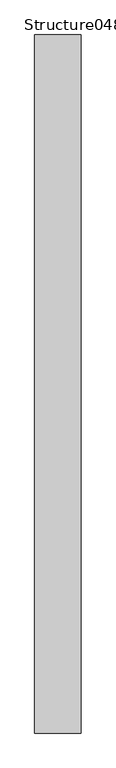
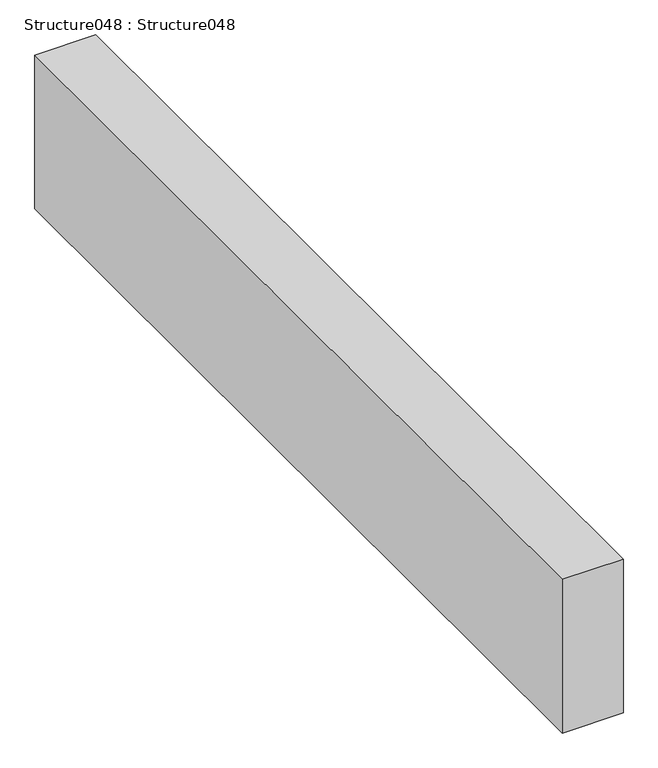
"""IFC4 building model written with IfcOpenShell, lengths in millimetres: proxy geometry, Structure048 : Structure048."""

from ifc_helpers import new_model, si_unit, frame, origin, place, context, project, spatial, polyline, outline, extrude, source, transform, mapped, element, save


def structure048_structure048_38ab66bb(model_context):
    return source(origin(), model_context, "Body", "SweptSolid", [
        extrude(outline(polyline([(-991.9364422, -1052.8906574), (-1125.2864422, -1052.8906574), (-1125.2864422, 947.1093426), (-991.9364422, 947.1093426), (-991.9364422, -1052.8906574)])), frame((0.0, 0.0, 42133.8036692), z_axis=(0.0, 0.0, 1.0), x_axis=(1.0, 0.0, 0.0)), (0.0, 0.0, 1.0), 355.6),
    ])


if __name__ == "__main__":
    model = new_model("IFC4")
    model_context = context("Model", 3, world=origin())
    ifc_project = project(units=[si_unit("LENGTHUNIT", "METRE", prefix="MILLI")], contexts=[model_context])
    site = spatial("IfcSite", under=ifc_project)
    building = spatial("IfcBuilding", under=site)
    placement = place(None, origin())
    structure048_structure048_shape = structure048_structure048_38ab66bb(model_context)
    element("IfcBuildingElementProxy", 1, Name="Structure048 : Structure048", ObjectType="Structure048 : Structure048", at=placement, inside=building, context=model_context, shape_type="MappedRepresentation", body=[
        mapped(structure048_structure048_shape, transform((0.0, 0.0, 0.0), x_axis=(1.0, 0.0, 0.0), y_axis=(0.0, 1.0, 0.0), z_axis=(0.0, 0.0, 1.0))),
    ])
    save(model, "model.ifc")

# Revit data of these elements
# Type "Structure048 : Structure048"
#   NameOverride = "Structure048"
# Element 1 (IfcBuildingElementProxy, "Structure048 : Structure048")
#   Materials on its faces: "STRUCTURAL MEMBER (SEE STRUCTURAL DWGS)"
# Materials
#   "STRUCTURAL MEMBER (SEE STRUCTURAL DWGS)": class "Unassigned", colour RGB 176 134 95, transparency 0, Cost = 0
